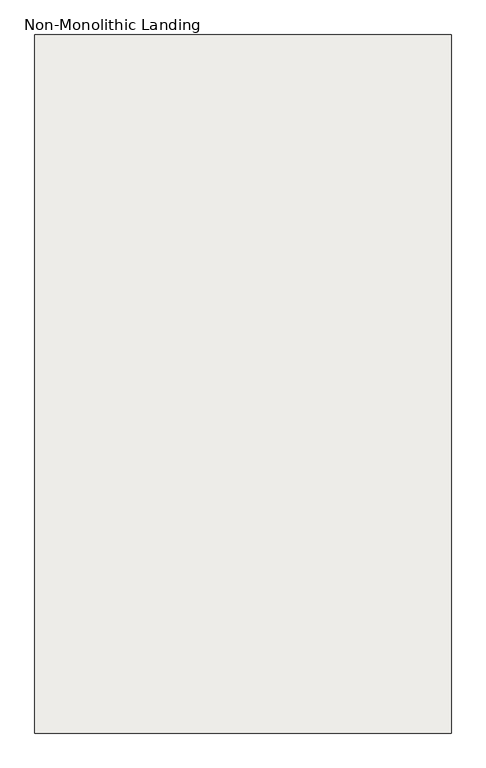
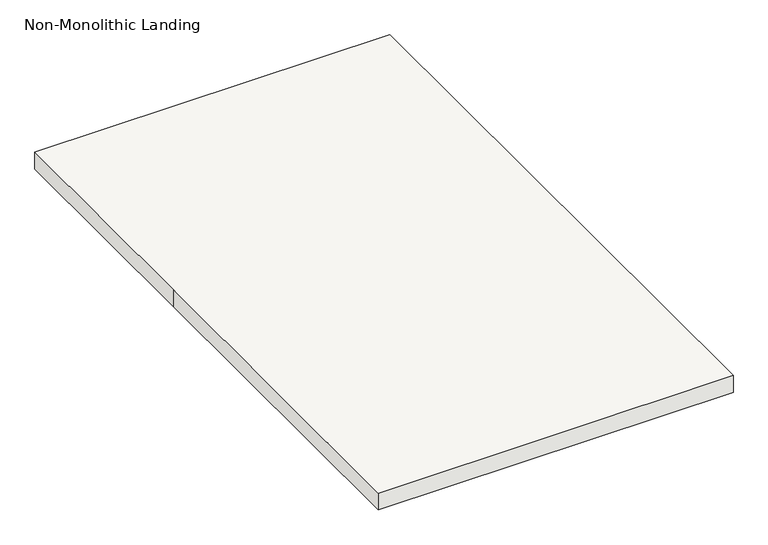
"""IFC4 building model written with IfcOpenShell, lengths in millimetres: slab geometry, Non-Monolithic Landing."""

from ifc_helpers import new_model, si_unit, frame, origin, place, context, project, spatial, polyline, outline, extrude, source, transform, mapped, element, save


def non_monolithic_landing_d44a62f3(model_context):
    return source(origin(), model_context, "Body", "SweptSolid", [
        extrude(outline(polyline([(21549.836337, -3576.2808257), (21549.836337, -2900.524372), (22549.836337, -2900.524372), (22549.836337, -4576.2808257), (21549.836337, -4576.2808257), (21549.836337, -3576.2808257)])), frame((0.0, 0.0, 1859.0909091), z_axis=(0.0, 0.0, 1.0), x_axis=(1.0, 0.0, 0.0)), (0.0, 0.0, 1.0), 50.0),
    ])


if __name__ == "__main__":
    model = new_model("IFC4")
    model_context = context("Model", 3, world=origin())
    ifc_project = project(units=[si_unit("LENGTHUNIT", "METRE", prefix="MILLI")], contexts=[model_context])
    site = spatial("IfcSite", under=ifc_project)
    building = spatial("IfcBuilding", under=site)
    placement = place(None, origin())
    non_monolithic_landing_shape = non_monolithic_landing_d44a62f3(model_context)
    element("IfcSlab", 1, ObjectType="Non-Monolithic Landing", at=placement, inside=building, context=model_context, shape_type="MappedRepresentation", body=[
        mapped(non_monolithic_landing_shape, transform((0.0, 0.0, 0.0), x_axis=(1.0, 0.0, 0.0), y_axis=(0.0, 1.0, 0.0), z_axis=(0.0, 0.0, 1.0))),
    ])
    save(model, "model.ifc")
